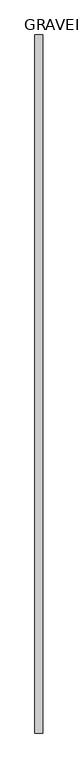
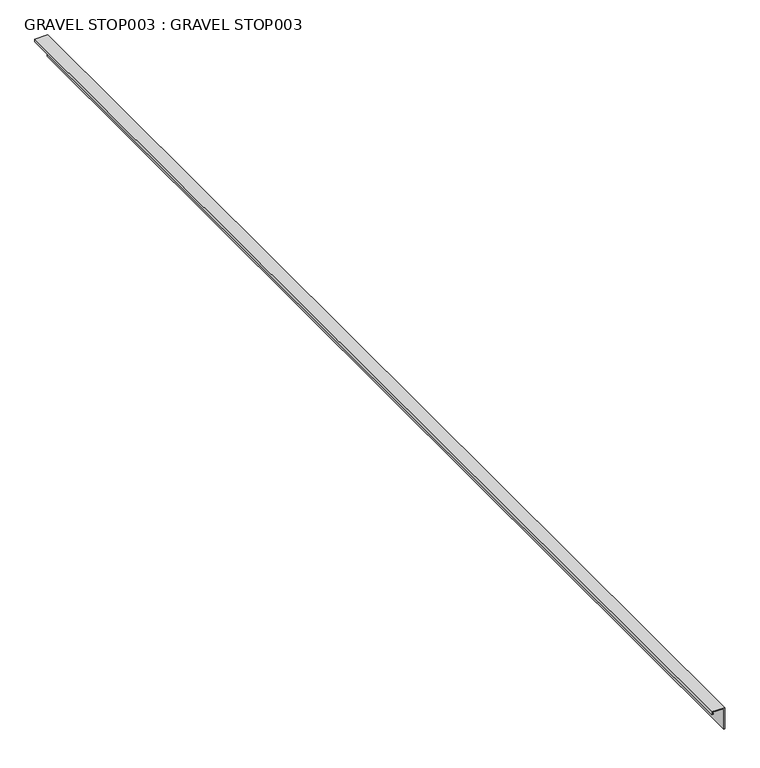
"""IFC4 building model written with IfcOpenShell, lengths in millimetres: proxy geometry, GRAVEL STOP003 : GRAVEL STOP003."""

from ifc_helpers import new_model, si_unit, frame, origin, place, context, project, spatial, polyline, outline, extrude, source, transform, mapped, element, save


def gravel_stop003_gravel_stop003_12768274(model_context):
    return source(origin(), model_context, "Body", "SweptSolid", [
        extrude(outline(polyline([(40234.4061757, -5021.258828), (40197.5761757, -5021.258828), (40197.5761757, -5019.988828), (40235.6761757, -5019.988828), (40235.6761757, -5042.213828), (40230.9263757, -5042.213828), (40230.9263757, -5039.2113716), (40232.1963757, -5039.2113716), (40232.1963757, -5040.943828), (40234.4061757, -5040.943828), (40234.4061757, -5021.258828)])), frame((0.0, -1052.8906573, 0.0), z_axis=(0.0, 1.0, 0.0), x_axis=(0.0, 0.0, 1.0)), (0.0, 0.0, 1.0), 2000.25),
    ])


if __name__ == "__main__":
    model = new_model("IFC4")
    model_context = context("Model", 3, world=origin())
    ifc_project = project(units=[si_unit("LENGTHUNIT", "METRE", prefix="MILLI")], contexts=[model_context])
    site = spatial("IfcSite", under=ifc_project)
    building = spatial("IfcBuilding", under=site)
    placement = place(None, origin())
    gravel_stop003_gravel_stop003_shape = gravel_stop003_gravel_stop003_12768274(model_context)
    element("IfcBuildingElementProxy", 1, Name="GRAVEL STOP003 : GRAVEL STOP003", ObjectType="GRAVEL STOP003 : GRAVEL STOP003", at=placement, inside=building, context=model_context, shape_type="MappedRepresentation", body=[
        mapped(gravel_stop003_gravel_stop003_shape, transform((0.0, 0.0, 0.0), x_axis=(1.0, 0.0, 0.0), y_axis=(0.0, 1.0, 0.0), z_axis=(0.0, 0.0, 1.0))),
    ])
    save(model, "model.ifc")

# Revit data of these elements
# Type "GRAVEL STOP003 : GRAVEL STOP003"
#   NameOverride = "GRAVEL STOP003"
# Element 1 (IfcBuildingElementProxy, "GRAVEL STOP003 : GRAVEL STOP003")
#   Materials on its faces: "COPPER STUCCO J BEAD"
# Materials
#   "COPPER STUCCO J BEAD": class "Unassigned", colour RGB 251 232 155, transparency 0, Cost = 0
